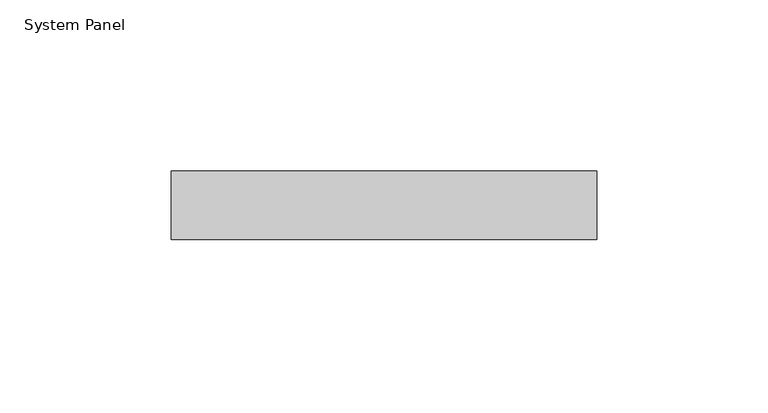
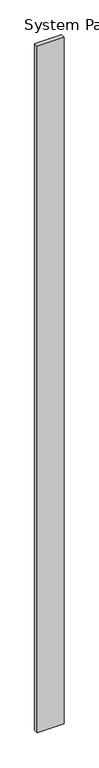
"""IFC4 building model written with IfcOpenShell, lengths in millimetres: plate geometry, System Panel : WWm-Glass-20mm-10mmOffset."""

import ifcopenshell
import ifcopenshell.guid

model = None  # the IFC model being written
_history = None  # IfcOwnerHistory: only IFC2X3 demands one
_inside = {}  # id of a spatial element -> (the spatial element, [elements in it])
_under = {}  # id of a project, library or spatial element -> (it, [spatial elements below it])
_declared = {}  # id of a project -> (the project, [libraries it declares])
_typed = {}  # id of a type object -> (the type object, [elements of that type])
_made_of = {}  # id of a material, layer set ... -> (it, [elements and type objects made of it])


def new_model(schema):
    """Start an empty IFC model of exactly this schema.

    Asked for "IFC4X3", IfcOpenShell would pick the latest addendum, in which some entities
    have other attributes; the version numbers below select the first issue.
    IFC2X3 requires an IfcOwnerHistory on every rooted entity: one is made here for all.
    """
    global model, _history
    if schema == "IFC4X3":
        model = ifcopenshell.file(schema_version=(4, 3, 0, 0))
    else:
        model = ifcopenshell.file(schema=schema)
    _inside.clear()
    _under.clear()
    _declared.clear()
    _typed.clear()
    _made_of.clear()
    _history = None
    if model.schema == "IFC2X3":
        org = make("IfcOrganization", Name="unknown")
        user = make(
            "IfcPersonAndOrganization",
            ThePerson=make("IfcPerson", FamilyName="unknown"),
            TheOrganization=org,
        )
        app = make(
            "IfcApplication",
            ApplicationDeveloper=org,
            Version="unknown",
            ApplicationFullName="unknown",
            ApplicationIdentifier="unknown",
        )
        _history = make(
            "IfcOwnerHistory",
            OwningUser=user,
            OwningApplication=app,
            ChangeAction="ADDED",
            CreationDate=0,
        )
    return model


def make(cls, **values):
    """One entity of the class cls with the attributes given. An attribute that is None is left unset."""
    return model.create_entity(
        cls, **{name: value for name, value in values.items() if value is not None}
    )


def rooted(cls, **values):
    """An entity with a GlobalId (a new one), such as an element, a storey or a relation."""
    return make(cls, GlobalId=ifcopenshell.guid.new(), OwnerHistory=_history, **values)


def si_unit(unit_type, name, prefix=None):
    """IfcSIUnit, for example si_unit("LENGTHUNIT", "METRE", prefix="MILLI")."""
    return make("IfcSIUnit", UnitType=unit_type, Prefix=prefix, Name=name)


def assignment(units):
    """IfcUnitAssignment: the units of a project."""
    return None if units is None else make("IfcUnitAssignment", Units=units)


def point(xyz):
    """IfcCartesianPoint."""
    return None if xyz is None else make("IfcCartesianPoint", Coordinates=xyz)


def direction(xyz):
    """IfcDirection."""
    return None if xyz is None else make("IfcDirection", DirectionRatios=xyz)


def frame(location, z_axis=None, x_axis=None):
    """IfcAxis2Placement3D, a coordinate frame: its origin and axes. An axis left out is left unset."""
    return make(
        "IfcAxis2Placement3D",
        Location=point(location),
        Axis=direction(z_axis),
        RefDirection=direction(x_axis),
    )


def origin():
    """The frame at (0, 0, 0) with its axes left unset."""
    return frame((0.0, 0.0, 0.0))


def origin_with_axes():
    """The frame at (0, 0, 0) with the z axis (0, 0, 1) and the x axis (1, 0, 0) written out."""
    return frame((0.0, 0.0, 0.0), z_axis=(0.0, 0.0, 1.0), x_axis=(1.0, 0.0, 0.0))


def place(relative_to, where):
    """IfcLocalPlacement: puts the frame where relative to a parent placement (None: the world)."""
    return make(
        "IfcLocalPlacement", PlacementRelTo=relative_to, RelativePlacement=where
    )


def context(
    kind, dimensions, precision=None, world=None, true_north=None, identifier=None
):
    """IfcGeometricRepresentationContext, for example the 3D "Model" context."""
    return make(
        "IfcGeometricRepresentationContext",
        ContextIdentifier=identifier,
        ContextType=kind,
        CoordinateSpaceDimension=dimensions,
        Precision=precision,
        WorldCoordinateSystem=world,
        TrueNorth=true_north,
    )


def project(units=None, contexts=None):
    """IfcProject with its units and contexts."""
    return rooted(
        "IfcProject",
        Name="project",
        RepresentationContexts=contexts,
        UnitsInContext=assignment(units),
    )


def spatial(cls, under=None, at=None, **own):
    """A site, building, storey or space (cls), placed at a placement, below another one or the project."""
    s = rooted(cls, ObjectPlacement=at, **own)
    if under is not None:
        _under.setdefault(under.id(), (under, []))[1].append(s)
    return s


def polyline(points):
    """IfcPolyline through the points."""
    return make("IfcPolyline", Points=[point(p) for p in points])


def outline(outer, holes=None, kind="AREA"):
    """IfcArbitraryClosedProfileDef: a profile drawn as a closed curve; with holes, ...WithVoids."""
    if holes is None:
        return make("IfcArbitraryClosedProfileDef", ProfileType=kind, OuterCurve=outer)
    return make(
        "IfcArbitraryProfileDefWithVoids",
        ProfileType=kind,
        OuterCurve=outer,
        InnerCurves=holes,
    )


def extrude(swept, where, along, depth):
    """IfcExtrudedAreaSolid: the profile swept, set in the frame where, extruded along a direction by depth."""
    return make(
        "IfcExtrudedAreaSolid",
        SweptArea=swept,
        Position=where,
        ExtrudedDirection=direction(along),
        Depth=depth,
    )


def shape(context_of_items, identifier, shape_type, items):
    """IfcShapeRepresentation: the items that make up one representation, for example the "Body"."""
    return make(
        "IfcShapeRepresentation",
        ContextOfItems=context_of_items,
        RepresentationIdentifier=identifier,
        RepresentationType=shape_type,
        Items=items,
    )


def source(mapping_origin, context_of_items, identifier, shape_type, items):
    """IfcRepresentationMap: a shape defined once, which mapped items show again and again."""
    return make(
        "IfcRepresentationMap",
        MappingOrigin=mapping_origin,
        MappedRepresentation=shape(context_of_items, identifier, shape_type, items),
    )


def transform(
    local_origin,
    x_axis=None,
    y_axis=None,
    z_axis=None,
    scale=None,
    scale2=None,
    scale3=None,
    uniform=True,
):
    """IfcCartesianTransformationOperator3D, or its non-uniform kind. x_axis, y_axis, z_axis: its Axis1, 2, 3."""
    if uniform:
        return make(
            "IfcCartesianTransformationOperator3D",
            Axis1=direction(x_axis),
            Axis2=direction(y_axis),
            LocalOrigin=point(local_origin),
            Scale=scale,
            Axis3=direction(z_axis),
        )
    return make(
        "IfcCartesianTransformationOperator3DnonUniform",
        Axis1=direction(x_axis),
        Axis2=direction(y_axis),
        LocalOrigin=point(local_origin),
        Scale=scale,
        Axis3=direction(z_axis),
        Scale2=scale2,
        Scale3=scale3,
    )


def mapped(mapping_source, mapping_target):
    """IfcMappedItem: shows the shape of a source again, moved by a transform."""
    return make(
        "IfcMappedItem", MappingSource=mapping_source, MappingTarget=mapping_target
    )


def made_of(thing, what):
    """Note that an element or type object is made of a material, layer set ...; save() writes the relation."""
    if what is not None:
        _made_of.setdefault(what.id(), (what, []))[1].append(thing)
    return thing


def element(
    cls,
    number,
    at=None,
    inside=None,
    cuts=None,
    type_object=None,
    material=None,
    context=None,
    identifier="Body",
    shape_type=None,
    held_by="IfcProductDefinitionShape",
    body=None,
    shapes=None,
    **own,
):
    """One element of the class cls, such as IfcWall. Its Tag is "e" and its number.

    at: its placement. inside: the storey or other place that contains it. cuts: it is an
    opening in that element (IfcRelVoidsElement). A single representation is given by context,
    identifier, shape_type and body (its items); several are given by shapes. held_by: the class
    of the entity that holds the representations. save() writes the other relations.
    """
    e = rooted(cls, Tag="e%d" % number, ObjectPlacement=at, **own)
    if body is not None:
        shapes = [shape(context, identifier, shape_type, body)]
    if shapes is not None:
        e.Representation = make(held_by, Representations=shapes)
    if inside is not None:
        _inside.setdefault(inside.id(), (inside, []))[1].append(e)
    if cuts is not None:
        rooted(
            "IfcRelVoidsElement", RelatingBuildingElement=cuts, RelatedOpeningElement=e
        )
    if type_object is not None:
        _typed.setdefault(type_object.id(), (type_object, []))[1].append(e)
    return made_of(e, material)


def aggregate(whole, parts):
    """IfcRelAggregates: a whole, such as a stair, and the parts it consists of."""
    return rooted("IfcRelAggregates", RelatingObject=whole, RelatedObjects=parts)


def save(model, path):
    """Write the relations noted so far, then the file.

    IfcRelAggregates (storeys below a building ...), IfcRelContainedInSpatialStructure (elements
    in a storey), IfcRelDefinesByType, IfcRelAssociatesMaterial and IfcRelDeclares: one each for
    every whole, place, type object, material and project.
    """
    for whole, parts in _under.values():
        aggregate(whole, parts)
    for where, things in _inside.values():
        rooted(
            "IfcRelContainedInSpatialStructure",
            RelatedElements=things,
            RelatingStructure=where,
        )
    for kind, things in _typed.values():
        rooted("IfcRelDefinesByType", RelatedObjects=things, RelatingType=kind)
    for what, things in _made_of.values():
        rooted("IfcRelAssociatesMaterial", RelatedObjects=things, RelatingMaterial=what)
    for by, libraries in _declared.values():
        rooted("IfcRelDeclares", RelatingContext=by, RelatedDefinitions=libraries)
    model.write(path)


def system_panel_9dcbbef9(model_context):
    return source(origin(), model_context, "Body", "SweptSolid", [
        extrude(outline(polyline([(62.0040329, 0.0), (-62.0040329, 0.0), (-62.0040329, 20.0), (62.0040329, 20.0), (62.0040329, 0.0)])), origin_with_axes(), (0.0, 0.0, 1.0), 3350.0),
    ])


if __name__ == "__main__":
    model = new_model("IFC4")
    model_context = context("Model", 3, world=origin())
    ifc_project = project(units=[si_unit("LENGTHUNIT", "METRE", prefix="MILLI")], contexts=[model_context])
    site = spatial("IfcSite", under=ifc_project)
    building = spatial("IfcBuilding", under=site)
    placement = place(None, origin())
    system_panel_shape = system_panel_9dcbbef9(model_context)
    element("IfcPlate", 1, ObjectType="System Panel : WWm-Glass-20mm-10mmOffset", at=placement, inside=building, context=model_context, shape_type="MappedRepresentation", body=[
        mapped(system_panel_shape, transform((0.0, 0.0, 0.0), x_axis=(1.0, 0.0, 0.0), y_axis=(0.0, 1.0, 0.0), z_axis=(0.0, 0.0, 1.0))),
    ])
    save(model, "model.ifc")

# Revit data of these elements
# Type "System Panel : WWm-Glass-20mm-10mmOffset"
#   Finish = ""
# Element 1 (IfcPlate, "System Panel : WWm-Glass-20mm-10mmOffset")
#   Materials on its faces: "WW-EC-GL-Storefront"
# Materials
#   "WW-EC-GL-Storefront": class "Glass", colour RGB 236 240 239, transparency 0.85, Description = "Storefront Glass", Cost = 0
